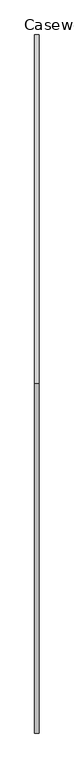
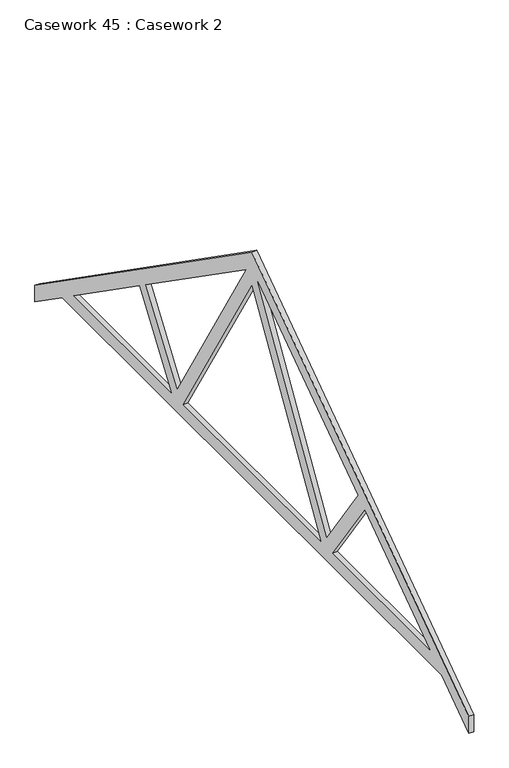
"""IFC4 building model written with IfcOpenShell, lengths in millimetres: furniture geometry, Casework 45 : Casework 2."""

from ifc_helpers import new_model, si_unit, frame, origin, place, context, project, spatial, polyline, outline, extrude, source, transform, mapped, element, save


def casework_45_casework_2_a6fc9b56(model_context):
    return source(origin(), model_context, "Body", "SweptSolid", [
        extrude(outline(polyline([(6583.1149316, 5250.0), (-277.3850684, 5250.0), (-767.3850684, 4906.8983063), (-767.3850684, 5090.0144946), (3152.8649316, 7835.0030963), (7073.1149316, 5090.0144946), (7073.1149316, 4906.8983063), (6583.1149316, 5250.0)]), holes=[polyline([(4612.3149663, 5400.0), (6368.8927306, 5400.0), (5190.2113591, 6225.3215815), (4612.3149663, 5400.0)]), polyline([(4394.2037684, 5400.0), (3152.8649316, 7465.9347567), (1911.5260948, 5400.0), (4394.2037684, 5400.0)]), polyline([(4504.5438357, 5507.6038939), (5067.3385525, 6311.3580469), (3262.0771677, 7575.415677), (4504.5438357, 5507.6038939)]), polyline([(1693.4148969, 5400.0), (1115.5185041, 6225.3215815), (-63.1628674, 5400.0), (1693.4148969, 5400.0)]), polyline([(1801.1860276, 5507.6038939), (3043.6526956, 7575.415677), (1238.3913108, 6311.3580469), (1801.1860276, 5507.6038939)])]), frame((-9821.5247381, 0.0, 0.0), z_axis=(1.0, 0.0, 0.0), x_axis=(0.0, 1.0, 0.0)), (0.0, 0.0, 1.0), 49.6351915),
    ])


if __name__ == "__main__":
    model = new_model("IFC4")
    model_context = context("Model", 3, world=origin())
    ifc_project = project(units=[si_unit("LENGTHUNIT", "METRE", prefix="MILLI")], contexts=[model_context])
    site = spatial("IfcSite", under=ifc_project)
    building = spatial("IfcBuilding", under=site)
    placement = place(None, origin())
    casework_45_casework_2_shape = casework_45_casework_2_a6fc9b56(model_context)
    element("IfcFurniture", 1, ObjectType="Casework 45 : Casework 2", at=placement, inside=building, context=model_context, shape_type="MappedRepresentation", body=[
        mapped(casework_45_casework_2_shape, transform((0.0, 0.0, 0.0), x_axis=(1.0, 0.0, 0.0), y_axis=(0.0, 1.0, 0.0), z_axis=(0.0, 0.0, 1.0))),
    ])
    save(model, "model.ifc")

# Revit data of these elements
# Element 1 (IfcFurniture, "Casework 45 : Casework 2")
#   Materials on its faces: "Softwood, Lumber"
# Materials
#   "Softwood, Lumber": class "Wood", colour RGB 205 156 65, transparency 0, Description = "Pinus Echinata", Cost = 0
